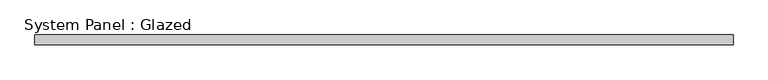
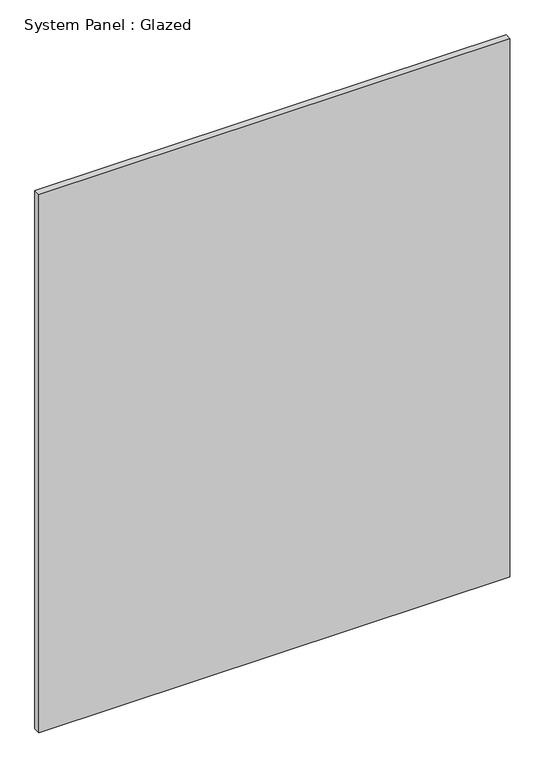
"""IFC4 building model written with IfcOpenShell, lengths in millimetres: plate geometry, System Panel : Glazed."""

import ifcopenshell
import ifcopenshell.guid

model = None  # the IFC model being written
_history = None  # IfcOwnerHistory: only IFC2X3 demands one
_inside = {}  # id of a spatial element -> (the spatial element, [elements in it])
_under = {}  # id of a project, library or spatial element -> (it, [spatial elements below it])
_declared = {}  # id of a project -> (the project, [libraries it declares])
_typed = {}  # id of a type object -> (the type object, [elements of that type])
_made_of = {}  # id of a material, layer set ... -> (it, [elements and type objects made of it])


def new_model(schema):
    """Start an empty IFC model of exactly this schema.

    Asked for "IFC4X3", IfcOpenShell would pick the latest addendum, in which some entities
    have other attributes; the version numbers below select the first issue.
    IFC2X3 requires an IfcOwnerHistory on every rooted entity: one is made here for all.
    """
    global model, _history
    if schema == "IFC4X3":
        model = ifcopenshell.file(schema_version=(4, 3, 0, 0))
    else:
        model = ifcopenshell.file(schema=schema)
    _inside.clear()
    _under.clear()
    _declared.clear()
    _typed.clear()
    _made_of.clear()
    _history = None
    if model.schema == "IFC2X3":
        org = make("IfcOrganization", Name="unknown")
        user = make(
            "IfcPersonAndOrganization",
            ThePerson=make("IfcPerson", FamilyName="unknown"),
            TheOrganization=org,
        )
        app = make(
            "IfcApplication",
            ApplicationDeveloper=org,
            Version="unknown",
            ApplicationFullName="unknown",
            ApplicationIdentifier="unknown",
        )
        _history = make(
            "IfcOwnerHistory",
            OwningUser=user,
            OwningApplication=app,
            ChangeAction="ADDED",
            CreationDate=0,
        )
    return model


def make(cls, **values):
    """One entity of the class cls with the attributes given. An attribute that is None is left unset."""
    return model.create_entity(
        cls, **{name: value for name, value in values.items() if value is not None}
    )


def rooted(cls, **values):
    """An entity with a GlobalId (a new one), such as an element, a storey or a relation."""
    return make(cls, GlobalId=ifcopenshell.guid.new(), OwnerHistory=_history, **values)


def si_unit(unit_type, name, prefix=None):
    """IfcSIUnit, for example si_unit("LENGTHUNIT", "METRE", prefix="MILLI")."""
    return make("IfcSIUnit", UnitType=unit_type, Prefix=prefix, Name=name)


def assignment(units):
    """IfcUnitAssignment: the units of a project."""
    return None if units is None else make("IfcUnitAssignment", Units=units)


def point(xyz):
    """IfcCartesianPoint."""
    return None if xyz is None else make("IfcCartesianPoint", Coordinates=xyz)


def direction(xyz):
    """IfcDirection."""
    return None if xyz is None else make("IfcDirection", DirectionRatios=xyz)


def frame(location, z_axis=None, x_axis=None):
    """IfcAxis2Placement3D, a coordinate frame: its origin and axes. An axis left out is left unset."""
    return make(
        "IfcAxis2Placement3D",
        Location=point(location),
        Axis=direction(z_axis),
        RefDirection=direction(x_axis),
    )


def origin():
    """The frame at (0, 0, 0) with its axes left unset."""
    return frame((0.0, 0.0, 0.0))


def origin_with_axes():
    """The frame at (0, 0, 0) with the z axis (0, 0, 1) and the x axis (1, 0, 0) written out."""
    return frame((0.0, 0.0, 0.0), z_axis=(0.0, 0.0, 1.0), x_axis=(1.0, 0.0, 0.0))


def place(relative_to, where):
    """IfcLocalPlacement: puts the frame where relative to a parent placement (None: the world)."""
    return make(
        "IfcLocalPlacement", PlacementRelTo=relative_to, RelativePlacement=where
    )


def context(
    kind, dimensions, precision=None, world=None, true_north=None, identifier=None
):
    """IfcGeometricRepresentationContext, for example the 3D "Model" context."""
    return make(
        "IfcGeometricRepresentationContext",
        ContextIdentifier=identifier,
        ContextType=kind,
        CoordinateSpaceDimension=dimensions,
        Precision=precision,
        WorldCoordinateSystem=world,
        TrueNorth=true_north,
    )


def project(units=None, contexts=None):
    """IfcProject with its units and contexts."""
    return rooted(
        "IfcProject",
        Name="project",
        RepresentationContexts=contexts,
        UnitsInContext=assignment(units),
    )


def spatial(cls, under=None, at=None, **own):
    """A site, building, storey or space (cls), placed at a placement, below another one or the project."""
    s = rooted(cls, ObjectPlacement=at, **own)
    if under is not None:
        _under.setdefault(under.id(), (under, []))[1].append(s)
    return s


def polyline(points):
    """IfcPolyline through the points."""
    return make("IfcPolyline", Points=[point(p) for p in points])


def outline(outer, holes=None, kind="AREA"):
    """IfcArbitraryClosedProfileDef: a profile drawn as a closed curve; with holes, ...WithVoids."""
    if holes is None:
        return make("IfcArbitraryClosedProfileDef", ProfileType=kind, OuterCurve=outer)
    return make(
        "IfcArbitraryProfileDefWithVoids",
        ProfileType=kind,
        OuterCurve=outer,
        InnerCurves=holes,
    )


def extrude(swept, where, along, depth):
    """IfcExtrudedAreaSolid: the profile swept, set in the frame where, extruded along a direction by depth."""
    return make(
        "IfcExtrudedAreaSolid",
        SweptArea=swept,
        Position=where,
        ExtrudedDirection=direction(along),
        Depth=depth,
    )


def shape(context_of_items, identifier, shape_type, items):
    """IfcShapeRepresentation: the items that make up one representation, for example the "Body"."""
    return make(
        "IfcShapeRepresentation",
        ContextOfItems=context_of_items,
        RepresentationIdentifier=identifier,
        RepresentationType=shape_type,
        Items=items,
    )


def source(mapping_origin, context_of_items, identifier, shape_type, items):
    """IfcRepresentationMap: a shape defined once, which mapped items show again and again."""
    return make(
        "IfcRepresentationMap",
        MappingOrigin=mapping_origin,
        MappedRepresentation=shape(context_of_items, identifier, shape_type, items),
    )


def transform(
    local_origin,
    x_axis=None,
    y_axis=None,
    z_axis=None,
    scale=None,
    scale2=None,
    scale3=None,
    uniform=True,
):
    """IfcCartesianTransformationOperator3D, or its non-uniform kind. x_axis, y_axis, z_axis: its Axis1, 2, 3."""
    if uniform:
        return make(
            "IfcCartesianTransformationOperator3D",
            Axis1=direction(x_axis),
            Axis2=direction(y_axis),
            LocalOrigin=point(local_origin),
            Scale=scale,
            Axis3=direction(z_axis),
        )
    return make(
        "IfcCartesianTransformationOperator3DnonUniform",
        Axis1=direction(x_axis),
        Axis2=direction(y_axis),
        LocalOrigin=point(local_origin),
        Scale=scale,
        Axis3=direction(z_axis),
        Scale2=scale2,
        Scale3=scale3,
    )


def mapped(mapping_source, mapping_target):
    """IfcMappedItem: shows the shape of a source again, moved by a transform."""
    return make(
        "IfcMappedItem", MappingSource=mapping_source, MappingTarget=mapping_target
    )


def made_of(thing, what):
    """Note that an element or type object is made of a material, layer set ...; save() writes the relation."""
    if what is not None:
        _made_of.setdefault(what.id(), (what, []))[1].append(thing)
    return thing


def element(
    cls,
    number,
    at=None,
    inside=None,
    cuts=None,
    type_object=None,
    material=None,
    context=None,
    identifier="Body",
    shape_type=None,
    held_by="IfcProductDefinitionShape",
    body=None,
    shapes=None,
    **own,
):
    """One element of the class cls, such as IfcWall. Its Tag is "e" and its number.

    at: its placement. inside: the storey or other place that contains it. cuts: it is an
    opening in that element (IfcRelVoidsElement). A single representation is given by context,
    identifier, shape_type and body (its items); several are given by shapes. held_by: the class
    of the entity that holds the representations. save() writes the other relations.
    """
    e = rooted(cls, Tag="e%d" % number, ObjectPlacement=at, **own)
    if body is not None:
        shapes = [shape(context, identifier, shape_type, body)]
    if shapes is not None:
        e.Representation = make(held_by, Representations=shapes)
    if inside is not None:
        _inside.setdefault(inside.id(), (inside, []))[1].append(e)
    if cuts is not None:
        rooted(
            "IfcRelVoidsElement", RelatingBuildingElement=cuts, RelatedOpeningElement=e
        )
    if type_object is not None:
        _typed.setdefault(type_object.id(), (type_object, []))[1].append(e)
    return made_of(e, material)


def aggregate(whole, parts):
    """IfcRelAggregates: a whole, such as a stair, and the parts it consists of."""
    return rooted("IfcRelAggregates", RelatingObject=whole, RelatedObjects=parts)


def save(model, path):
    """Write the relations noted so far, then the file.

    IfcRelAggregates (storeys below a building ...), IfcRelContainedInSpatialStructure (elements
    in a storey), IfcRelDefinesByType, IfcRelAssociatesMaterial and IfcRelDeclares: one each for
    every whole, place, type object, material and project.
    """
    for whole, parts in _under.values():
        aggregate(whole, parts)
    for where, things in _inside.values():
        rooted(
            "IfcRelContainedInSpatialStructure",
            RelatedElements=things,
            RelatingStructure=where,
        )
    for kind, things in _typed.values():
        rooted("IfcRelDefinesByType", RelatedObjects=things, RelatingType=kind)
    for what, things in _made_of.values():
        rooted("IfcRelAssociatesMaterial", RelatedObjects=things, RelatingMaterial=what)
    for by, libraries in _declared.values():
        rooted("IfcRelDeclares", RelatingContext=by, RelatedDefinitions=libraries)
    model.write(path)


def system_panel_glazed_aeb7b79b(model_context):
    return source(origin(), model_context, "Body", "SweptSolid", [
        extrude(outline(polyline([(879.5, -49.5), (-879.5, -49.5), (-879.5, -24.5), (879.5, -24.5), (879.5, -49.5)])), origin_with_axes(), (0.0, 0.0, 1.0), 2125.0),
    ])


if __name__ == "__main__":
    model = new_model("IFC4")
    model_context = context("Model", 3, world=origin())
    ifc_project = project(units=[si_unit("LENGTHUNIT", "METRE", prefix="MILLI")], contexts=[model_context])
    site = spatial("IfcSite", under=ifc_project)
    building = spatial("IfcBuilding", under=site)
    placement = place(None, origin())
    system_panel_glazed_shape = system_panel_glazed_aeb7b79b(model_context)
    element("IfcPlate", 1, ObjectType="System Panel : Glazed", at=placement, inside=building, context=model_context, shape_type="MappedRepresentation", body=[
        mapped(system_panel_glazed_shape, transform((0.0, 0.0, 0.0), x_axis=(1.0, 0.0, 0.0), y_axis=(0.0, 1.0, 0.0), z_axis=(0.0, 0.0, 1.0))),
    ])
    save(model, "model.ifc")

# Revit data of these elements
# Type "System Panel : Glazed"
#   Keynote = "H11"
#   Construction Type Id = "GSP4R"
#   Analytic Construction = "1/8 in Pilkington single glazing"
#   Visual Light Transmittance = 0.9
#   Solar Heat Gain Coefficient = 0.86
#   Heat Transfer Coefficient (U) = 6.7069 W/(m²·K)
# Element 1 (IfcPlate, "System Panel : Glazed")
#   Materials on its faces: "Glass"
# Materials
#   "Glass": class "Glass", colour RGB 0 128 192, transparency 0.9, Description = "Soda Lime Glass", Cost = 0
